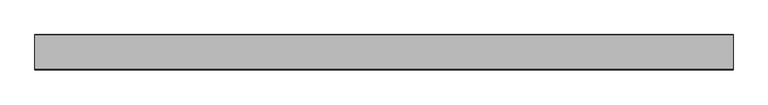
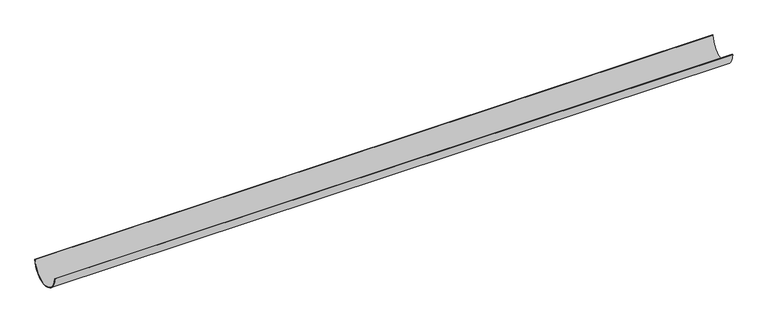
"""IFC4 building model written with IfcOpenShell, lengths in millimetres: proxy geometry, TN_ПВС 125-82_Водосточный желоб : TN_ПВС 125-82_Водосточный желоб."""

from ifc_helpers import new_model, si_unit, point, frame, origin, origin_2d, place, context, project, spatial, polyline, circle_curve, trimmed, segment, composite_curve, outline, extrude, source, transform, mapped, element, save


def generic_models_1bbf0373(model_context):
    return source(origin(), model_context, "Body", "SweptSolid", [
        extrude(outline(composite_curve([segment(trimmed(circle_curve(origin_2d(), 76.1), [point((76.1, 0.0))], [point((-76.1, 0.0))], False, "CARTESIAN"), True, "CONTINUOUS"), segment(polyline([(-76.1, 0.0), (-74.1, 0.0)]), True, "CONTINUOUS"), segment(trimmed(circle_curve(origin_2d(), 74.1), [point((-74.1, 0.0))], [point((74.1, 0.0))], True, "CARTESIAN"), True, "CONTINUOUS"), segment(polyline([(74.1, 0.0), (76.1, 0.0)]), True, "CONTINUOUS")], self_intersect=False)), frame((0.0, 0.0, 0.0), z_axis=(1.0, 0.0, 0.0), x_axis=(0.0, 1.0, 0.0)), (0.0, 0.0, 1.0), 3000.0),
    ])


if __name__ == "__main__":
    model = new_model("IFC4")
    model_context = context("Model", 3, world=origin())
    ifc_project = project(units=[si_unit("LENGTHUNIT", "METRE", prefix="MILLI")], contexts=[model_context])
    site = spatial("IfcSite", under=ifc_project)
    building = spatial("IfcBuilding", under=site)
    placement = place(None, origin())
    generic_models_shape = generic_models_1bbf0373(model_context)
    element("IfcBuildingElementProxy", 1, Name="TN_ПВС 125-82_Водосточный желоб : TN_ПВС 125-82_Водосточный желоб", ObjectType="TN_ПВС 125-82_Водосточный желоб : TN_ПВС 125-82_Водосточный желоб", at=placement, inside=building, context=model_context, shape_type="MappedRepresentation", body=[
        mapped(generic_models_shape, transform((0.0, 0.0, 0.0), x_axis=(1.0, 0.0, 0.0), y_axis=(0.0, 1.0, 0.0), z_axis=(0.0, 0.0, 1.0))),
    ])
    save(model, "model.ifc")

# Revit data of these elements
# Type "TN_ПВС 125-82_Водосточный желоб : TN_ПВС 125-82_Водосточный желоб"
#   Description = "Предназначен для сбора дождевой\r\nи талой воды с кровли."
#   Manufacturer = "ТехноНИКОЛЬ"
#   Model = "Комплектующие к водосточным системам"
#   URL = "https://tn-vodostok.ru/catalog/pvh/"
#   ADSK_Обозначение = "ТехноНИКОЛЬ"
#   ADSK_Наименование краткое = "Желоб"
#   ADSK_Наименование = "Водосточный желоб"
#   ADSK_Масса_Текст = ""
#   ADSK_Марка = ""
#   ADSK_Код изделия = ""
#   ADSK_Завод-изготовитель = "ТехноНИКОЛЬ"
#   ADSK_Единица измерения = "п.м."
#   ADSK_Группирование = "Комплектующие к водосточным системам"
#   ADSK_URL страницы изделия = "https://tn-vodostok.ru/catalog/pvh/"
#   ADSK_URL документации изделия = "https://tn-vodostok.ru/upload/iblock/c42/c427963cb77eb5c3c51f0cfb870e9e52.pdf"
#   ADSK_Размер_Длина [instance default] = 500 mm
#   ADSK_Количество [instance default] = 0.5
#   ADSK_Материал [instance default] = TN_Пластик_Коричневый_RAL8019
#   Default Elevation = 0
# Element 1 (IfcBuildingElementProxy, "TN_ПВС 125-82_Водосточный желоб : TN_ПВС 125-82_Водосточный желоб")
#   ADSK_Размер_Длина = 3000 mm
#   ADSK_Количество = 3
#   Materials on its faces: "TN_Пластик_Коричневый_RAL8019"
# Materials
#   "TN_Пластик_Коричневый_RAL8019": class "Типовые", colour RGB 61 54 53, transparency 0, Cost = 0
